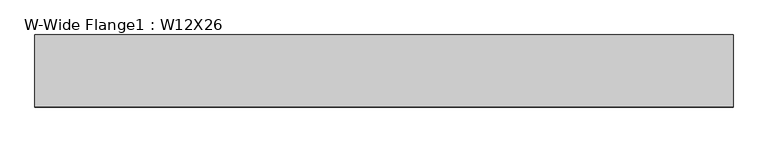
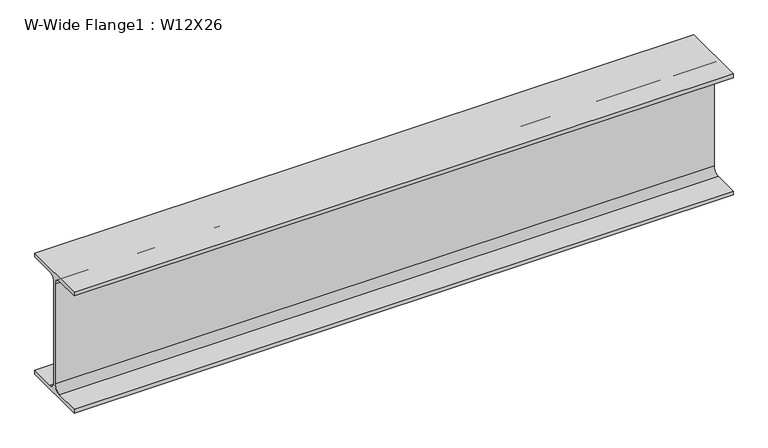
"""IFC4 building model written with IfcOpenShell, lengths in millimetres: beam geometry, W-Wide Flange1 : W12X26."""

import ifcopenshell
import ifcopenshell.guid

model = None  # the IFC model being written
_history = None  # IfcOwnerHistory: only IFC2X3 demands one
_inside = {}  # id of a spatial element -> (the spatial element, [elements in it])
_under = {}  # id of a project, library or spatial element -> (it, [spatial elements below it])
_declared = {}  # id of a project -> (the project, [libraries it declares])
_typed = {}  # id of a type object -> (the type object, [elements of that type])
_made_of = {}  # id of a material, layer set ... -> (it, [elements and type objects made of it])


def new_model(schema):
    """Start an empty IFC model of exactly this schema.

    Asked for "IFC4X3", IfcOpenShell would pick the latest addendum, in which some entities
    have other attributes; the version numbers below select the first issue.
    IFC2X3 requires an IfcOwnerHistory on every rooted entity: one is made here for all.
    """
    global model, _history
    if schema == "IFC4X3":
        model = ifcopenshell.file(schema_version=(4, 3, 0, 0))
    else:
        model = ifcopenshell.file(schema=schema)
    _inside.clear()
    _under.clear()
    _declared.clear()
    _typed.clear()
    _made_of.clear()
    _history = None
    if model.schema == "IFC2X3":
        org = make("IfcOrganization", Name="unknown")
        user = make(
            "IfcPersonAndOrganization",
            ThePerson=make("IfcPerson", FamilyName="unknown"),
            TheOrganization=org,
        )
        app = make(
            "IfcApplication",
            ApplicationDeveloper=org,
            Version="unknown",
            ApplicationFullName="unknown",
            ApplicationIdentifier="unknown",
        )
        _history = make(
            "IfcOwnerHistory",
            OwningUser=user,
            OwningApplication=app,
            ChangeAction="ADDED",
            CreationDate=0,
        )
    return model


def make(cls, **values):
    """One entity of the class cls with the attributes given. An attribute that is None is left unset."""
    return model.create_entity(
        cls, **{name: value for name, value in values.items() if value is not None}
    )


def rooted(cls, **values):
    """An entity with a GlobalId (a new one), such as an element, a storey or a relation."""
    return make(cls, GlobalId=ifcopenshell.guid.new(), OwnerHistory=_history, **values)


def si_unit(unit_type, name, prefix=None):
    """IfcSIUnit, for example si_unit("LENGTHUNIT", "METRE", prefix="MILLI")."""
    return make("IfcSIUnit", UnitType=unit_type, Prefix=prefix, Name=name)


def assignment(units):
    """IfcUnitAssignment: the units of a project."""
    return None if units is None else make("IfcUnitAssignment", Units=units)


def point(xyz):
    """IfcCartesianPoint."""
    return None if xyz is None else make("IfcCartesianPoint", Coordinates=xyz)


def direction(xyz):
    """IfcDirection."""
    return None if xyz is None else make("IfcDirection", DirectionRatios=xyz)


def frame(location, z_axis=None, x_axis=None):
    """IfcAxis2Placement3D, a coordinate frame: its origin and axes. An axis left out is left unset."""
    return make(
        "IfcAxis2Placement3D",
        Location=point(location),
        Axis=direction(z_axis),
        RefDirection=direction(x_axis),
    )


def frame_2d(location, x_axis=None):
    """IfcAxis2Placement2D, a coordinate frame in the plane: its origin and x axis."""
    return make(
        "IfcAxis2Placement2D", Location=point(location), RefDirection=direction(x_axis)
    )


def origin():
    """The frame at (0, 0, 0) with its axes left unset."""
    return frame((0.0, 0.0, 0.0))


def place(relative_to, where):
    """IfcLocalPlacement: puts the frame where relative to a parent placement (None: the world)."""
    return make(
        "IfcLocalPlacement", PlacementRelTo=relative_to, RelativePlacement=where
    )


def context(
    kind, dimensions, precision=None, world=None, true_north=None, identifier=None
):
    """IfcGeometricRepresentationContext, for example the 3D "Model" context."""
    return make(
        "IfcGeometricRepresentationContext",
        ContextIdentifier=identifier,
        ContextType=kind,
        CoordinateSpaceDimension=dimensions,
        Precision=precision,
        WorldCoordinateSystem=world,
        TrueNorth=true_north,
    )


def project(units=None, contexts=None):
    """IfcProject with its units and contexts."""
    return rooted(
        "IfcProject",
        Name="project",
        RepresentationContexts=contexts,
        UnitsInContext=assignment(units),
    )


def spatial(cls, under=None, at=None, **own):
    """A site, building, storey or space (cls), placed at a placement, below another one or the project."""
    s = rooted(cls, ObjectPlacement=at, **own)
    if under is not None:
        _under.setdefault(under.id(), (under, []))[1].append(s)
    return s


def polyline(points):
    """IfcPolyline through the points."""
    return make("IfcPolyline", Points=[point(p) for p in points])


def circle_curve(where, radius):
    """IfcCircle in the frame where."""
    return make("IfcCircle", Position=where, Radius=radius)


def trimmed(basis, trim1, trim2, sense, master):
    """IfcTrimmedCurve: the piece of a basis curve between two trims."""
    return make(
        "IfcTrimmedCurve",
        BasisCurve=basis,
        Trim1=trim1,
        Trim2=trim2,
        SenseAgreement=sense,
        MasterRepresentation=master,
    )


def segment(curve, same_sense, transition):
    """IfcCompositeCurveSegment."""
    return make(
        "IfcCompositeCurveSegment",
        Transition=transition,
        SameSense=same_sense,
        ParentCurve=curve,
    )


def composite_curve(segments, self_intersect=None):
    """IfcCompositeCurve: segments joined end to end."""
    return make("IfcCompositeCurve", Segments=segments, SelfIntersect=self_intersect)


def outline(outer, holes=None, kind="AREA"):
    """IfcArbitraryClosedProfileDef: a profile drawn as a closed curve; with holes, ...WithVoids."""
    if holes is None:
        return make("IfcArbitraryClosedProfileDef", ProfileType=kind, OuterCurve=outer)
    return make(
        "IfcArbitraryProfileDefWithVoids",
        ProfileType=kind,
        OuterCurve=outer,
        InnerCurves=holes,
    )


def extrude(swept, where, along, depth):
    """IfcExtrudedAreaSolid: the profile swept, set in the frame where, extruded along a direction by depth."""
    return make(
        "IfcExtrudedAreaSolid",
        SweptArea=swept,
        Position=where,
        ExtrudedDirection=direction(along),
        Depth=depth,
    )


def shape(context_of_items, identifier, shape_type, items):
    """IfcShapeRepresentation: the items that make up one representation, for example the "Body"."""
    return make(
        "IfcShapeRepresentation",
        ContextOfItems=context_of_items,
        RepresentationIdentifier=identifier,
        RepresentationType=shape_type,
        Items=items,
    )


def source(mapping_origin, context_of_items, identifier, shape_type, items):
    """IfcRepresentationMap: a shape defined once, which mapped items show again and again."""
    return make(
        "IfcRepresentationMap",
        MappingOrigin=mapping_origin,
        MappedRepresentation=shape(context_of_items, identifier, shape_type, items),
    )


def transform(
    local_origin,
    x_axis=None,
    y_axis=None,
    z_axis=None,
    scale=None,
    scale2=None,
    scale3=None,
    uniform=True,
):
    """IfcCartesianTransformationOperator3D, or its non-uniform kind. x_axis, y_axis, z_axis: its Axis1, 2, 3."""
    if uniform:
        return make(
            "IfcCartesianTransformationOperator3D",
            Axis1=direction(x_axis),
            Axis2=direction(y_axis),
            LocalOrigin=point(local_origin),
            Scale=scale,
            Axis3=direction(z_axis),
        )
    return make(
        "IfcCartesianTransformationOperator3DnonUniform",
        Axis1=direction(x_axis),
        Axis2=direction(y_axis),
        LocalOrigin=point(local_origin),
        Scale=scale,
        Axis3=direction(z_axis),
        Scale2=scale2,
        Scale3=scale3,
    )


def mapped(mapping_source, mapping_target):
    """IfcMappedItem: shows the shape of a source again, moved by a transform."""
    return make(
        "IfcMappedItem", MappingSource=mapping_source, MappingTarget=mapping_target
    )


def made_of(thing, what):
    """Note that an element or type object is made of a material, layer set ...; save() writes the relation."""
    if what is not None:
        _made_of.setdefault(what.id(), (what, []))[1].append(thing)
    return thing


def element(
    cls,
    number,
    at=None,
    inside=None,
    cuts=None,
    type_object=None,
    material=None,
    context=None,
    identifier="Body",
    shape_type=None,
    held_by="IfcProductDefinitionShape",
    body=None,
    shapes=None,
    **own,
):
    """One element of the class cls, such as IfcWall. Its Tag is "e" and its number.

    at: its placement. inside: the storey or other place that contains it. cuts: it is an
    opening in that element (IfcRelVoidsElement). A single representation is given by context,
    identifier, shape_type and body (its items); several are given by shapes. held_by: the class
    of the entity that holds the representations. save() writes the other relations.
    """
    e = rooted(cls, Tag="e%d" % number, ObjectPlacement=at, **own)
    if body is not None:
        shapes = [shape(context, identifier, shape_type, body)]
    if shapes is not None:
        e.Representation = make(held_by, Representations=shapes)
    if inside is not None:
        _inside.setdefault(inside.id(), (inside, []))[1].append(e)
    if cuts is not None:
        rooted(
            "IfcRelVoidsElement", RelatingBuildingElement=cuts, RelatedOpeningElement=e
        )
    if type_object is not None:
        _typed.setdefault(type_object.id(), (type_object, []))[1].append(e)
    return made_of(e, material)


def aggregate(whole, parts):
    """IfcRelAggregates: a whole, such as a stair, and the parts it consists of."""
    return rooted("IfcRelAggregates", RelatingObject=whole, RelatedObjects=parts)


def save(model, path):
    """Write the relations noted so far, then the file.

    IfcRelAggregates (storeys below a building ...), IfcRelContainedInSpatialStructure (elements
    in a storey), IfcRelDefinesByType, IfcRelAssociatesMaterial and IfcRelDeclares: one each for
    every whole, place, type object, material and project.
    """
    for whole, parts in _under.values():
        aggregate(whole, parts)
    for where, things in _inside.values():
        rooted(
            "IfcRelContainedInSpatialStructure",
            RelatedElements=things,
            RelatingStructure=where,
        )
    for kind, things in _typed.values():
        rooted("IfcRelDefinesByType", RelatedObjects=things, RelatingType=kind)
    for what, things in _made_of.values():
        rooted("IfcRelAssociatesMaterial", RelatedObjects=things, RelatingMaterial=what)
    for by, libraries in _declared.values():
        rooted("IfcRelDeclares", RelatingContext=by, RelatedDefinitions=libraries)
    model.write(path)


def w_wide_flange1_w12x26_de2c28aa(model_context):
    return source(origin(), model_context, "Body", "SweptSolid", [
        extrude(outline(composite_curve([segment(polyline([(82.423, -145.288), (82.423, -154.94), (-82.423, -154.94), (-82.423, -145.288), (-20.2565, -145.288)]), True, "CONTINUOUS"), segment(trimmed(circle_curve(frame_2d((-20.2565, -127.9525)), 17.3355), [point((-20.2565, -145.288))], [point((-2.921, -127.9525))], True, "CARTESIAN"), True, "CONTINUOUS"), segment(polyline([(-2.921, -127.9525), (-2.921, 127.9525)]), True, "CONTINUOUS"), segment(trimmed(circle_curve(frame_2d((-20.2565, 127.9525)), 17.3355), [point((-2.921, 127.9525))], [point((-20.2565, 145.288))], True, "CARTESIAN"), True, "CONTINUOUS"), segment(polyline([(-20.2565, 145.288), (-82.423, 145.288), (-82.423, 154.94), (82.423, 154.94), (82.423, 145.288), (20.2565, 145.288)]), True, "CONTINUOUS"), segment(trimmed(circle_curve(frame_2d((20.2565, 127.9525)), 17.3355), [point((20.2565, 145.288))], [point((2.921, 127.9525))], True, "CARTESIAN"), True, "CONTINUOUS"), segment(polyline([(2.921, 127.9525), (2.921, -127.9525)]), True, "CONTINUOUS"), segment(trimmed(circle_curve(frame_2d((20.2565, -127.9525)), 17.3355), [point((2.921, -127.9525))], [point((20.2565, -145.288))], True, "CARTESIAN"), True, "CONTINUOUS"), segment(polyline([(20.2565, -145.288), (82.423, -145.288)]), True, "CONTINUOUS")], self_intersect=False)), frame((-750.1310059, 0.0, 0.0), z_axis=(1.0, 0.0, 0.0), x_axis=(0.0, 1.0, 0.0)), (0.0, 0.0, 1.0), 1596.7970771),
    ])


if __name__ == "__main__":
    model = new_model("IFC4")
    model_context = context("Model", 3, world=origin())
    ifc_project = project(units=[si_unit("LENGTHUNIT", "METRE", prefix="MILLI")], contexts=[model_context])
    site = spatial("IfcSite", under=ifc_project)
    building = spatial("IfcBuilding", under=site)
    placement = place(None, origin())
    w_wide_flange1_w12x26_shape = w_wide_flange1_w12x26_de2c28aa(model_context)
    element("IfcBeam", 1, ObjectType="W-Wide Flange1 : W12X26", at=placement, inside=building, context=model_context, shape_type="MappedRepresentation", body=[
        mapped(w_wide_flange1_w12x26_shape, transform((0.0, 0.0, 0.0), x_axis=(1.0, 0.0, 0.0), y_axis=(0.0, 1.0, 0.0), z_axis=(0.0, 0.0, 1.0))),
    ])
    save(model, "model.ifc")

# Revit data of these elements
# Type "W-Wide Flange1 : W12X26"
#   Assembly Code = "B10"
#   W = 26
#   Start Extension Calculation [instance default] = 10' - 0"
#   Start Extension [instance default] = -0' - 0 1/2"
#   End Extension Calculation [instance default] = 10' - 0"
#   End Extension [instance default] = -0' - 0 1/2"
#   Length [instance default] = 5' - 0"
#   bf = 0' - 6.49"
#   d = 1' - 0.2"
#   k = 0' - 1 1/16"
#   k2 = 0' - 0.6825"
#   tf = 0' - 0.38"
#   tw = 0' - 0.23"
#   A = 0.053125 SF
#   Structural Material [instance default] = Metal - Steel - ASTM A992
# Element 1 (IfcBeam, "W-Wide Flange1 : W12X26")
#   Materials on its faces: "Metal - Steel - ASTM A992"
# Materials
#   "Metal - Steel - ASTM A992": class "Metal", colour RGB 199 199 199, transparency 0
